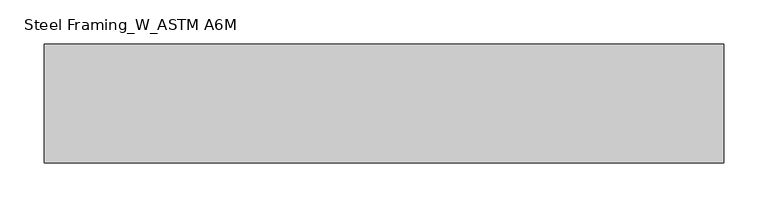
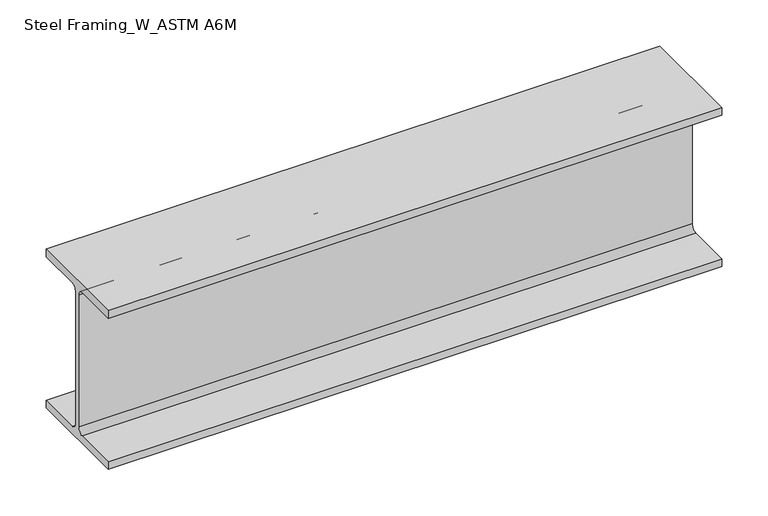
"""IFC4 building model written with IfcOpenShell, lengths in millimetres: beam geometry, Steel Framing_W_ASTM A6M : H_SB_AR_S02_W200x31.3_B6."""

from ifc_helpers import new_model, si_unit, point, frame, frame_2d, origin, place, context, project, spatial, polyline, circle_curve, trimmed, segment, composite_curve, outline, extrude, source, transform, mapped, element, save


def steel_framing_w_astm_a6m_53d98241(model_context):
    return source(origin(), model_context, "Body", "SweptSolid", [
        extrude(outline(composite_curve([segment(polyline([(67.0, -94.8), (67.0, -105.0), (-67.0, -105.0), (-67.0, -94.8), (-10.775, -94.8)]), True, "CONTINUOUS"), segment(trimmed(circle_curve(frame_2d((-10.775, -87.2)), 7.6), [point((-10.775, -94.8))], [point((-3.175, -87.2))], True, "CARTESIAN"), True, "CONTINUOUS"), segment(polyline([(-3.175, -87.2), (-3.175, 87.2)]), True, "CONTINUOUS"), segment(trimmed(circle_curve(frame_2d((-10.775, 87.2)), 7.6), [point((-3.175, 87.2))], [point((-10.775, 94.8))], True, "CARTESIAN"), True, "CONTINUOUS"), segment(polyline([(-10.775, 94.8), (-67.0, 94.8), (-67.0, 105.0), (67.0, 105.0), (67.0, 94.8), (10.775, 94.8)]), True, "CONTINUOUS"), segment(trimmed(circle_curve(frame_2d((10.775, 87.2)), 7.6), [point((10.775, 94.8))], [point((3.175, 87.2))], True, "CARTESIAN"), True, "CONTINUOUS"), segment(polyline([(3.175, 87.2), (3.175, -87.2)]), True, "CONTINUOUS"), segment(trimmed(circle_curve(frame_2d((10.775, -87.2)), 7.6), [point((3.175, -87.2))], [point((10.775, -94.8))], True, "CARTESIAN"), True, "CONTINUOUS"), segment(polyline([(10.775, -94.8), (67.0, -94.8)]), True, "CONTINUOUS")], self_intersect=False)), frame((-346.3, 0.0, 0.0), z_axis=(1.0, 0.0, 0.0), x_axis=(0.0, 1.0, 0.0)), (0.0, 0.0, 1.0), 766.6),
    ])


if __name__ == "__main__":
    model = new_model("IFC4")
    model_context = context("Model", 3, world=origin())
    ifc_project = project(units=[si_unit("LENGTHUNIT", "METRE", prefix="MILLI")], contexts=[model_context])
    site = spatial("IfcSite", under=ifc_project)
    building = spatial("IfcBuilding", under=site)
    placement = place(None, origin())
    steel_framing_w_astm_a6m_shape = steel_framing_w_astm_a6m_53d98241(model_context)
    element("IfcBeam", 1, ObjectType="Steel Framing_W_ASTM A6M : H_SB_AR_S02_W200x31.3_B6", at=placement, inside=building, context=model_context, shape_type="MappedRepresentation", body=[
        mapped(steel_framing_w_astm_a6m_shape, transform((0.0, 0.0, 0.0), x_axis=(1.0, 0.0, 0.0), y_axis=(0.0, 1.0, 0.0), z_axis=(0.0, 0.0, 1.0))),
    ])
    save(model, "model.ifc")

# Revit data of these elements
# Type "Steel Framing_W_ASTM A6M : H_SB_AR_S02_W200x31.3_B6"
#   Type Mark = "B6"
#   Section Name Key = "W8x21"
#   Width = 13.4 cm
#   Web Thickness = 0.635 cm
#   Web Fillet = 0.76 cm
#   Warping Constant = 40800.0 cm⁶
#   Torsional Moment of Inertia = 11.70 cm⁴
#   Section Area = 39.7 cm²
#   Plastic Modulus weak axis = 93.2 cm³
#   Plastic Modulus strong axis = 334.0 cm³
#   Perimeter = 0.93 m²/m
#   Nominal Weight = 31.30 kgf/m
#   Moment of Inertia weak axis = 407.00 cm⁴
#   Moment of Inertia strong axis = 3130.00 cm⁴
#   Height = 21.0 cm
#   Flange Thickness = 1.02 cm
#   Elastic Modulus weak axis = 60.8 cm³
#   Elastic Modulus strong axis = 298.0 cm³
#   Centroid Vertical = 10.5 cm
#   Centroid Horizontal = 6.7 cm
#   Length [instance default] = 1500 mm
#   Structural Material [instance default] = Steel, 45-345
#   Bolt Spacing = 0
#   Assembly Code = ""
# Element 1 (IfcBeam, "Steel Framing_W_ASTM A6M : H_SB_AR_S02_W200x31.3_B6")
#   Structural Material = Steel ASTM A36
#   Materials on its faces: "Steel ASTM A36"
# Materials
#   "Steel, 45-345": class "Metal", colour RGB 189 187 185, transparency 0, Description = "Steel 345 MPa", Cost = 0
#   "Steel ASTM A36": class "Metal", colour RGB 199 199 199, transparency 0, Description = "Structural steel, ASTM A36 Grade B, mill finish", Cost = 0
